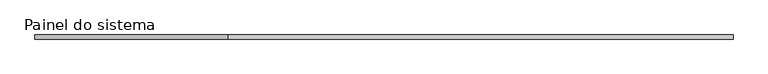
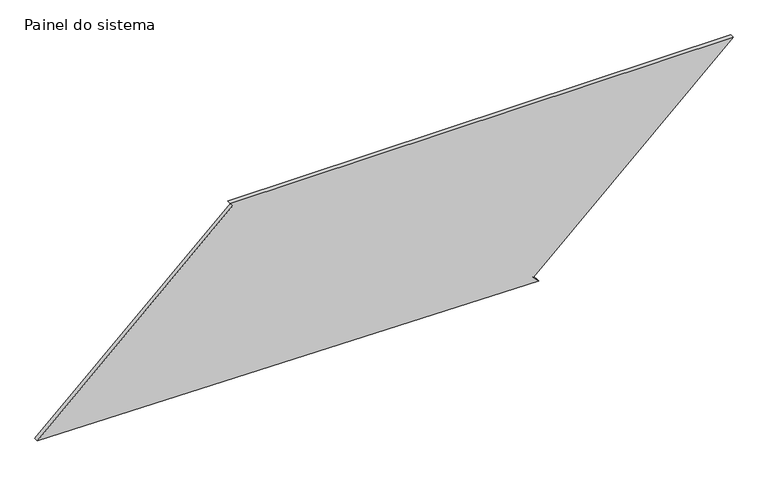
"""IFC4 building model written with IfcOpenShell, lengths in millimetres: plate geometry, Painel do sistema : Envidraçado."""

import ifcopenshell
import ifcopenshell.guid

model = None  # the IFC model being written
_history = None  # IfcOwnerHistory: only IFC2X3 demands one
_inside = {}  # id of a spatial element -> (the spatial element, [elements in it])
_under = {}  # id of a project, library or spatial element -> (it, [spatial elements below it])
_declared = {}  # id of a project -> (the project, [libraries it declares])
_typed = {}  # id of a type object -> (the type object, [elements of that type])
_made_of = {}  # id of a material, layer set ... -> (it, [elements and type objects made of it])


def new_model(schema):
    """Start an empty IFC model of exactly this schema.

    Asked for "IFC4X3", IfcOpenShell would pick the latest addendum, in which some entities
    have other attributes; the version numbers below select the first issue.
    IFC2X3 requires an IfcOwnerHistory on every rooted entity: one is made here for all.
    """
    global model, _history
    if schema == "IFC4X3":
        model = ifcopenshell.file(schema_version=(4, 3, 0, 0))
    else:
        model = ifcopenshell.file(schema=schema)
    _inside.clear()
    _under.clear()
    _declared.clear()
    _typed.clear()
    _made_of.clear()
    _history = None
    if model.schema == "IFC2X3":
        org = make("IfcOrganization", Name="unknown")
        user = make(
            "IfcPersonAndOrganization",
            ThePerson=make("IfcPerson", FamilyName="unknown"),
            TheOrganization=org,
        )
        app = make(
            "IfcApplication",
            ApplicationDeveloper=org,
            Version="unknown",
            ApplicationFullName="unknown",
            ApplicationIdentifier="unknown",
        )
        _history = make(
            "IfcOwnerHistory",
            OwningUser=user,
            OwningApplication=app,
            ChangeAction="ADDED",
            CreationDate=0,
        )
    return model


def make(cls, **values):
    """One entity of the class cls with the attributes given. An attribute that is None is left unset."""
    return model.create_entity(
        cls, **{name: value for name, value in values.items() if value is not None}
    )


def rooted(cls, **values):
    """An entity with a GlobalId (a new one), such as an element, a storey or a relation."""
    return make(cls, GlobalId=ifcopenshell.guid.new(), OwnerHistory=_history, **values)


def si_unit(unit_type, name, prefix=None):
    """IfcSIUnit, for example si_unit("LENGTHUNIT", "METRE", prefix="MILLI")."""
    return make("IfcSIUnit", UnitType=unit_type, Prefix=prefix, Name=name)


def assignment(units):
    """IfcUnitAssignment: the units of a project."""
    return None if units is None else make("IfcUnitAssignment", Units=units)


def point(xyz):
    """IfcCartesianPoint."""
    return None if xyz is None else make("IfcCartesianPoint", Coordinates=xyz)


def direction(xyz):
    """IfcDirection."""
    return None if xyz is None else make("IfcDirection", DirectionRatios=xyz)


def frame(location, z_axis=None, x_axis=None):
    """IfcAxis2Placement3D, a coordinate frame: its origin and axes. An axis left out is left unset."""
    return make(
        "IfcAxis2Placement3D",
        Location=point(location),
        Axis=direction(z_axis),
        RefDirection=direction(x_axis),
    )


def origin():
    """The frame at (0, 0, 0) with its axes left unset."""
    return frame((0.0, 0.0, 0.0))


def place(relative_to, where):
    """IfcLocalPlacement: puts the frame where relative to a parent placement (None: the world)."""
    return make(
        "IfcLocalPlacement", PlacementRelTo=relative_to, RelativePlacement=where
    )


def context(
    kind, dimensions, precision=None, world=None, true_north=None, identifier=None
):
    """IfcGeometricRepresentationContext, for example the 3D "Model" context."""
    return make(
        "IfcGeometricRepresentationContext",
        ContextIdentifier=identifier,
        ContextType=kind,
        CoordinateSpaceDimension=dimensions,
        Precision=precision,
        WorldCoordinateSystem=world,
        TrueNorth=true_north,
    )


def project(units=None, contexts=None):
    """IfcProject with its units and contexts."""
    return rooted(
        "IfcProject",
        Name="project",
        RepresentationContexts=contexts,
        UnitsInContext=assignment(units),
    )


def spatial(cls, under=None, at=None, **own):
    """A site, building, storey or space (cls), placed at a placement, below another one or the project."""
    s = rooted(cls, ObjectPlacement=at, **own)
    if under is not None:
        _under.setdefault(under.id(), (under, []))[1].append(s)
    return s


def polyline(points):
    """IfcPolyline through the points."""
    return make("IfcPolyline", Points=[point(p) for p in points])


def outline(outer, holes=None, kind="AREA"):
    """IfcArbitraryClosedProfileDef: a profile drawn as a closed curve; with holes, ...WithVoids."""
    if holes is None:
        return make("IfcArbitraryClosedProfileDef", ProfileType=kind, OuterCurve=outer)
    return make(
        "IfcArbitraryProfileDefWithVoids",
        ProfileType=kind,
        OuterCurve=outer,
        InnerCurves=holes,
    )


def extrude(swept, where, along, depth):
    """IfcExtrudedAreaSolid: the profile swept, set in the frame where, extruded along a direction by depth."""
    return make(
        "IfcExtrudedAreaSolid",
        SweptArea=swept,
        Position=where,
        ExtrudedDirection=direction(along),
        Depth=depth,
    )


def shape(context_of_items, identifier, shape_type, items):
    """IfcShapeRepresentation: the items that make up one representation, for example the "Body"."""
    return make(
        "IfcShapeRepresentation",
        ContextOfItems=context_of_items,
        RepresentationIdentifier=identifier,
        RepresentationType=shape_type,
        Items=items,
    )


def source(mapping_origin, context_of_items, identifier, shape_type, items):
    """IfcRepresentationMap: a shape defined once, which mapped items show again and again."""
    return make(
        "IfcRepresentationMap",
        MappingOrigin=mapping_origin,
        MappedRepresentation=shape(context_of_items, identifier, shape_type, items),
    )


def transform(
    local_origin,
    x_axis=None,
    y_axis=None,
    z_axis=None,
    scale=None,
    scale2=None,
    scale3=None,
    uniform=True,
):
    """IfcCartesianTransformationOperator3D, or its non-uniform kind. x_axis, y_axis, z_axis: its Axis1, 2, 3."""
    if uniform:
        return make(
            "IfcCartesianTransformationOperator3D",
            Axis1=direction(x_axis),
            Axis2=direction(y_axis),
            LocalOrigin=point(local_origin),
            Scale=scale,
            Axis3=direction(z_axis),
        )
    return make(
        "IfcCartesianTransformationOperator3DnonUniform",
        Axis1=direction(x_axis),
        Axis2=direction(y_axis),
        LocalOrigin=point(local_origin),
        Scale=scale,
        Axis3=direction(z_axis),
        Scale2=scale2,
        Scale3=scale3,
    )


def mapped(mapping_source, mapping_target):
    """IfcMappedItem: shows the shape of a source again, moved by a transform."""
    return make(
        "IfcMappedItem", MappingSource=mapping_source, MappingTarget=mapping_target
    )


def made_of(thing, what):
    """Note that an element or type object is made of a material, layer set ...; save() writes the relation."""
    if what is not None:
        _made_of.setdefault(what.id(), (what, []))[1].append(thing)
    return thing


def element(
    cls,
    number,
    at=None,
    inside=None,
    cuts=None,
    type_object=None,
    material=None,
    context=None,
    identifier="Body",
    shape_type=None,
    held_by="IfcProductDefinitionShape",
    body=None,
    shapes=None,
    **own,
):
    """One element of the class cls, such as IfcWall. Its Tag is "e" and its number.

    at: its placement. inside: the storey or other place that contains it. cuts: it is an
    opening in that element (IfcRelVoidsElement). A single representation is given by context,
    identifier, shape_type and body (its items); several are given by shapes. held_by: the class
    of the entity that holds the representations. save() writes the other relations.
    """
    e = rooted(cls, Tag="e%d" % number, ObjectPlacement=at, **own)
    if body is not None:
        shapes = [shape(context, identifier, shape_type, body)]
    if shapes is not None:
        e.Representation = make(held_by, Representations=shapes)
    if inside is not None:
        _inside.setdefault(inside.id(), (inside, []))[1].append(e)
    if cuts is not None:
        rooted(
            "IfcRelVoidsElement", RelatingBuildingElement=cuts, RelatedOpeningElement=e
        )
    if type_object is not None:
        _typed.setdefault(type_object.id(), (type_object, []))[1].append(e)
    return made_of(e, material)


def aggregate(whole, parts):
    """IfcRelAggregates: a whole, such as a stair, and the parts it consists of."""
    return rooted("IfcRelAggregates", RelatingObject=whole, RelatedObjects=parts)


def save(model, path):
    """Write the relations noted so far, then the file.

    IfcRelAggregates (storeys below a building ...), IfcRelContainedInSpatialStructure (elements
    in a storey), IfcRelDefinesByType, IfcRelAssociatesMaterial and IfcRelDeclares: one each for
    every whole, place, type object, material and project.
    """
    for whole, parts in _under.values():
        aggregate(whole, parts)
    for where, things in _inside.values():
        rooted(
            "IfcRelContainedInSpatialStructure",
            RelatedElements=things,
            RelatingStructure=where,
        )
    for kind, things in _typed.values():
        rooted("IfcRelDefinesByType", RelatedObjects=things, RelatingType=kind)
    for what, things in _made_of.values():
        rooted("IfcRelAssociatesMaterial", RelatedObjects=things, RelatingMaterial=what)
    for by, libraries in _declared.values():
        rooted("IfcRelDeclares", RelatingContext=by, RelatedDefinitions=libraries)
    model.write(path)


def painel_do_sistema_f64068f6(model_context):
    return source(origin(), model_context, "Body", "SweptSolid", [
        extrude(outline(polyline([(0.0, 940.9126061), (36.7529903, 907.0124924), (1163.9349836, 2129.0529027), (1163.9349836, -948.8944378), (1145.5584885, -931.9443809), (41.3730962, -2129.0529027), (0.0, 940.9126061)])), frame((0.0, 24.5, 0.0), z_axis=(0.0, 1.0, 0.0), x_axis=(0.0, 0.0, 1.0)), (0.0, 0.0, 1.0), 25.0),
    ])


if __name__ == "__main__":
    model = new_model("IFC4")
    model_context = context("Model", 3, world=origin())
    ifc_project = project(units=[si_unit("LENGTHUNIT", "METRE", prefix="MILLI")], contexts=[model_context])
    site = spatial("IfcSite", under=ifc_project)
    building = spatial("IfcBuilding", under=site)
    placement = place(None, origin())
    painel_do_sistema_shape = painel_do_sistema_f64068f6(model_context)
    element("IfcPlate", 1, ObjectType="Painel do sistema : Envidraçado", at=placement, inside=building, context=model_context, shape_type="MappedRepresentation", body=[
        mapped(painel_do_sistema_shape, transform((0.0, 0.0, 0.0), x_axis=(1.0, 0.0, 0.0), y_axis=(0.0, 1.0, 0.0), z_axis=(0.0, 0.0, 1.0))),
    ])
    save(model, "model.ifc")

# Revit data of these elements
# Type "Painel do sistema : Envidraçado"
#   Construction Type Id = "GSP4R"
#   Analytic Construction = "Vidraça única Pilkington 1/8 pol"
#   Visual Light Transmittance = 0.9
#   Solar Heat Gain Coefficient = 0.86
#   Heat Transfer Coefficient (U) = 6.7069 W/(m²·K)
# Element 1 (IfcPlate, "Painel do sistema : Envidraçado")
#   Materials on its faces: "Vidro"
# Materials
#   "Vidro": class "Vidro", colour RGB 0 128 192, transparency 0.9, Description = "Vidro de sílica", Cost = 0
